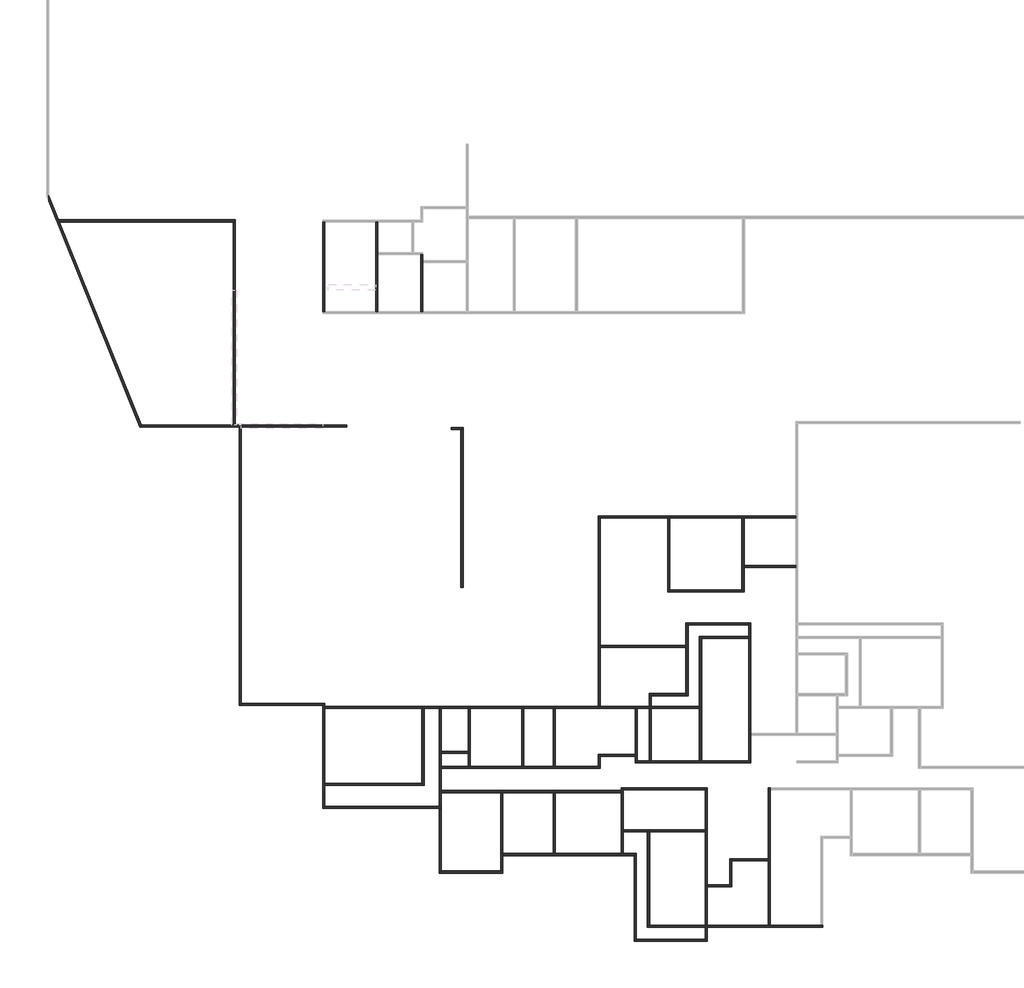
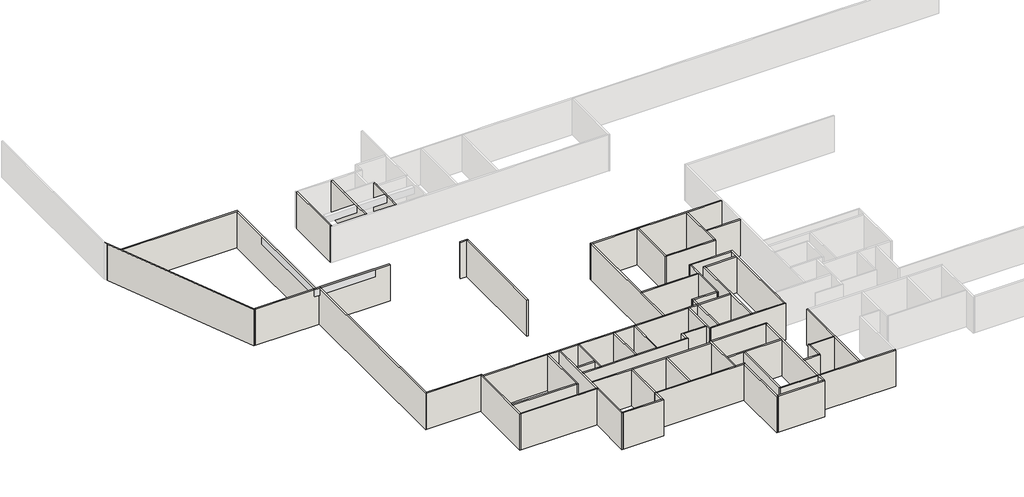
# One storey, part 1 of 8: 62 walls.
"""IFC4 building model written with IfcOpenShell, lengths in millimetres."""

from ifc_helpers import new_model, si_unit, origin, origin_with_axes, place, context, project, spatial, polyline, outline, extrude, faceted_brep, element, save

model = new_model("IFC4")

# Units and contexts
model_context = context("Model", 3, world=origin())
ifc_project = project(units=[si_unit("LENGTHUNIT", "METRE", prefix="MILLI")], contexts=[model_context])

# Site, building, storey
site = spatial("IfcSite", under=ifc_project)
building = spatial("IfcBuilding", under=site)
storey = spatial("IfcBuildingStorey", under=building, Name="户型图", Elevation=0.0)

# Walls
placement = place(None, origin())
element("IfcWall", 1, ObjectType="所有墙体", at=placement, inside=storey, context=model_context, shape_type="Brep", body=[
    faceted_brep([(85958.8477345, 57890.0043027, 0.0), (91177.79085, 44972.6668088, 0.0), (91177.79085, 44972.6668088, 3300.0), (85958.8477345, 57890.0043027, 3300.0), (85958.8477345, 58210.3403622, 0.0), (85958.8477345, 58210.3403622, 3300.0), (91258.731872, 45092.6668088, 3300.0), (91307.2150191, 44972.6668088, 3300.0), (91307.2150191, 44972.6668088, 0.0), (91258.731872, 45092.6668088, 0.0)], [[[0, 1, 2, 3]], [[4, 5, 6, 7, 8, 9]], [[1, 0, 4, 9, 8]], [[3, 2, 7, 6, 5]], [[0, 3, 5, 4]], [[2, 1, 8, 7]]]),
])
element("IfcWall", 2, ObjectType="所有墙体", at=placement, inside=storey, context=model_context, shape_type="Brep", body=[
    faceted_brep([(91307.2150191, 44972.6668088, 0.0), (96858.261361, 44972.6668088, 0.0), (96978.261361, 44972.6668088, 0.0), (96978.261361, 44972.6668088, 3300.0), (96858.261361, 44972.6668088, 3300.0), (96423.8477403, 44972.6668088, 3300.0), (91307.2150191, 44972.6668088, 3300.0), (91258.731872, 45092.6668088, 0.0), (91258.731872, 45092.6668088, 3300.0), (96723.8477403, 45092.6668088, 3300.0), (96978.261361, 45092.6668088, 3300.0), (96978.261361, 45092.6668088, 2700.0), (96978.261361, 45092.6668088, 0.0)], [[[0, 1, 2, 3, 4, 5, 6]], [[7, 8, 9, 10, 11, 12]], [[2, 1, 0, 7, 12]], [[6, 5, 4, 3, 10, 9, 8]], [[0, 6, 8, 7]], [[3, 2, 12, 11, 10]]]),
])
element("IfcWall", 3, ObjectType="所有墙体", at=placement, inside=storey, context=model_context, shape_type="Brep", body=[
    faceted_brep([(96858.261361, 44972.6668088, 0.0), (96858.261361, 29031.649632, 0.0), (96858.261361, 29031.649632, 3300.0), (96858.261361, 44882.6668088, 3300.0), (96858.261361, 44972.6668088, 3300.0), (96858.261361, 44972.6668088, 2700.0), (96978.261361, 44972.6668088, 0.0), (96978.261361, 44972.6668088, 3300.0), (96978.261361, 44882.6668088, 3300.0), (96978.261361, 29151.649632, 3300.0), (96978.261361, 29031.649632, 3300.0), (96978.261361, 29031.649632, 0.0), (96978.261361, 29151.649632, 0.0)], [[[0, 1, 2, 3, 4, 5]], [[6, 7, 8, 9, 10, 11, 12]], [[1, 0, 6, 12, 11]], [[4, 3, 2, 10, 9, 8, 7]], [[0, 5, 4, 7, 6]], [[2, 1, 11, 10]]]),
])
element("IfcWall", 4, ObjectType="所有墙体", at=placement, inside=storey, context=model_context, shape_type="Brep", body=[
    faceted_brep([(96978.261361, 29031.649632, 0.0), (101638.8477432, 29031.649632, 0.0), (101758.8477432, 29031.649632, 0.0), (101758.8477432, 29031.649632, 3300.0), (101638.8477432, 29031.649632, 3300.0), (96978.261361, 29031.649632, 3300.0), (96978.261361, 29151.649632, 0.0), (96978.261361, 29151.649632, 3300.0), (101648.7128309, 29151.649632, 3300.0), (101758.8477432, 29151.649632, 3300.0), (101758.8477432, 29151.649632, 2700.0), (101758.8477432, 29151.649632, 0.0)], [[[0, 1, 2, 3, 4, 5]], [[6, 7, 8, 9, 10, 11]], [[2, 1, 0, 6, 11]], [[5, 4, 3, 9, 8, 7]], [[0, 5, 7, 6]], [[3, 2, 11, 10, 9]]]),
])
element("IfcWall", 5, ObjectType="所有墙体", at=placement, inside=storey, context=model_context, shape_type="Brep", body=[
    faceted_brep([(101638.8477432, 29031.649632, 0.0), (101638.8477432, 23156.649475, 0.0), (101638.8477432, 23156.649475, 3300.0), (101638.8477432, 29031.649632, 3300.0), (101758.8477432, 29031.649632, 0.0), (101758.8477432, 29031.649632, 3300.0), (101758.8477432, 28766.8473862, 3300.0), (101758.8477432, 23276.649475, 3300.0), (101758.8477432, 23156.649475, 3300.0), (101758.8477432, 23156.649475, 0.0), (101758.8477432, 23276.649475, 0.0)], [[[0, 1, 2, 3]], [[4, 5, 6, 7, 8, 9, 10]], [[1, 0, 4, 10, 9]], [[3, 2, 8, 7, 6, 5]], [[0, 3, 5, 4]], [[2, 1, 9, 8]]]),
])
element("IfcWall", 6, ObjectType="所有墙体", at=placement, inside=storey, context=model_context, shape_type="Brep", body=[
    faceted_brep([(101758.8477432, 23156.649475, 0.0), (108307.9809936, 23156.649475, 0.0), (108427.9809936, 23156.649475, 0.0), (108427.9809936, 23156.649475, 3300.0), (108307.9809936, 23156.649475, 3300.0), (101758.8477432, 23156.649475, 3300.0), (101758.8477432, 23276.649475, 0.0), (101758.8477432, 23276.649475, 3300.0), (108427.9809936, 23276.649475, 3300.0), (108427.9809936, 23276.649475, 0.0)], [[[0, 1, 2, 3, 4, 5]], [[6, 7, 8, 9]], [[2, 1, 0, 6, 9]], [[5, 4, 3, 8, 7]], [[0, 5, 7, 6]], [[3, 2, 9, 8]]]),
])
element("IfcWall", 7, ObjectType="所有墙体", at=placement, inside=storey, context=model_context, shape_type="Brep", body=[
    faceted_brep([(108307.9809936, 23156.649475, 0.0), (108307.9809936, 19445.6854089, 0.0), (108307.9809936, 19445.6854089, 3300.0), (108307.9809936, 23156.649475, 3300.0), (108427.9809936, 23156.649475, 0.0), (108427.9809936, 23156.649475, 3300.0), (108427.9809936, 19565.6854089, 3300.0), (108427.9809936, 19445.6854089, 3300.0), (108427.9809936, 19445.6854089, 0.0), (108427.9809936, 19565.6854089, 0.0)], [[[0, 1, 2, 3]], [[4, 5, 6, 7, 8, 9]], [[1, 0, 4, 9, 8]], [[3, 2, 7, 6, 5]], [[0, 3, 5, 4]], [[2, 1, 8, 7]]]),
])
element("IfcWall", 8, ObjectType="所有墙体", at=placement, inside=storey, context=model_context, shape_type="Brep", body=[
    faceted_brep([(108427.9809936, 19445.6854089, 0.0), (111927.9809917, 19445.6854089, 0.0), (111927.9809917, 19445.6854089, 3300.0), (108427.9809936, 19445.6854089, 3300.0), (108427.9809936, 19565.6854089, 0.0), (108427.9809936, 19565.6854089, 3300.0), (111807.9809917, 19565.6854089, 3300.0), (111927.9809917, 19565.6854089, 3300.0), (111927.9809917, 19565.6854089, 0.0), (111807.9809917, 19565.6854089, 0.0)], [[[0, 1, 2, 3]], [[4, 5, 6, 7, 8, 9]], [[1, 0, 4, 9, 8]], [[3, 2, 7, 6, 5]], [[0, 3, 5, 4]], [[2, 1, 8, 7]]]),
])
element("IfcWall", 9, ObjectType="所有墙体", at=placement, inside=storey, context=model_context, shape_type="Brep", body=[
    faceted_brep([(111927.9809917, 19565.6854089, 0.0), (111927.9809917, 20445.6854086, 0.0), (111927.9809917, 20565.6854086, 0.0), (111927.9809917, 20565.6854086, 3300.0), (111927.9809917, 20445.6854086, 3300.0), (111927.9809917, 19565.6854089, 3300.0), (111807.9809917, 19565.6854089, 0.0), (111807.9809917, 19565.6854089, 3300.0), (111807.9809917, 20565.6854086, 3300.0), (111807.9809917, 20565.6854086, 0.0)], [[[0, 1, 2, 3, 4, 5]], [[6, 7, 8, 9]], [[2, 1, 0, 6, 9]], [[5, 4, 3, 8, 7]], [[0, 5, 7, 6]], [[3, 2, 9, 8]]]),
])
element("IfcWall", 10, ObjectType="所有墙体", at=placement, inside=storey, context=model_context, shape_type="Brep", body=[
    faceted_brep([(111927.9809917, 20445.6854086, 0.0), (119457.980985, 20445.6854086, 0.0), (119577.980985, 20445.6854086, 0.0), (119577.980985, 20445.6854086, 3300.0), (119457.980985, 20445.6854086, 3300.0), (111927.9809917, 20445.6854086, 3300.0), (111927.9809917, 20565.6854086, 0.0), (111927.9809917, 20565.6854086, 3300.0), (119577.980985, 20565.6854086, 3300.0), (119577.980985, 20565.6854086, 0.0)], [[[0, 1, 2, 3, 4, 5]], [[6, 7, 8, 9]], [[2, 1, 0, 6, 9]], [[5, 4, 3, 8, 7]], [[0, 5, 7, 6]], [[3, 2, 9, 8]]]),
])
element("IfcWall", 11, ObjectType="所有墙体", at=placement, inside=storey, context=model_context, shape_type="Brep", body=[
    faceted_brep([(119457.980985, 20445.6854086, 0.0), (119457.980985, 15545.6854122, 0.0), (119457.980985, 15545.6854122, 3300.0), (119457.980985, 20445.6854086, 3300.0), (119577.980985, 20445.6854086, 0.0), (119577.980985, 20445.6854086, 3300.0), (119577.980985, 15665.6854122, 3300.0), (119577.980985, 15545.6854122, 3300.0), (119577.980985, 15545.6854122, 0.0), (119577.980985, 15665.6854122, 0.0)], [[[0, 1, 2, 3]], [[4, 5, 6, 7, 8, 9]], [[1, 0, 4, 9, 8]], [[3, 2, 7, 6, 5]], [[0, 3, 5, 4]], [[2, 1, 8, 7]]]),
])
element("IfcWall", 12, ObjectType="所有墙体", at=placement, inside=storey, context=model_context, shape_type="Brep", body=[
    faceted_brep([(119577.980985, 15545.6854122, 0.0), (123627.9809864, 15545.6854122, 0.0), (123627.9809864, 15545.6854122, 3300.0), (119577.980985, 15545.6854122, 3300.0), (119577.980985, 15665.6854122, 0.0), (119577.980985, 15665.6854122, 3300.0), (123507.9809864, 15665.6854122, 3300.0), (123627.9809864, 15665.6854122, 3300.0), (123627.9809864, 15665.6854122, 0.0), (123507.9809864, 15665.6854122, 0.0)], [[[0, 1, 2, 3]], [[4, 5, 6, 7, 8, 9]], [[1, 0, 4, 9, 8]], [[3, 2, 7, 6, 5]], [[0, 3, 5, 4]], [[2, 1, 8, 7]]]),
])
element("IfcWall", 13, ObjectType="所有墙体", at=placement, inside=storey, context=model_context, shape_type="Brep", body=[
    faceted_brep([(123627.9809864, 15665.6854122, 0.0), (123627.9809864, 16345.6854162, 0.0), (123627.9809864, 16465.6854162, 0.0), (123627.9809864, 16465.6854162, 3300.0), (123627.9809864, 16345.6854162, 3300.0), (123627.9809864, 15665.6854122, 3300.0), (123507.9809864, 15665.6854122, 0.0), (123507.9809864, 15665.6854122, 3300.0), (123507.9809864, 16465.6854162, 3300.0), (123507.9809864, 16465.6854162, 0.0)], [[[0, 1, 2, 3, 4, 5]], [[6, 7, 8, 9]], [[2, 1, 0, 6, 9]], [[5, 4, 3, 8, 7]], [[0, 5, 7, 6]], [[3, 2, 9, 8]]]),
])
element("IfcWall", 14, ObjectType="所有墙体", at=placement, inside=storey, context=model_context, shape_type="Brep", body=[
    faceted_brep([(123627.9809864, 16345.6854162, 0.0), (130227.9809927, 16345.6854162, 0.0), (130227.9809927, 16345.6854162, 3300.0), (123627.9809864, 16345.6854162, 3300.0), (123627.9809864, 16465.6854162, 0.0), (123627.9809864, 16465.6854162, 3300.0), (130107.9809927, 16465.6854162, 3300.0), (130227.9809927, 16465.6854162, 3300.0), (130227.9809927, 16465.6854162, 0.0), (130107.9809927, 16465.6854162, 0.0)], [[[0, 1, 2, 3]], [[4, 5, 6, 7, 8, 9]], [[1, 0, 4, 9, 8]], [[3, 2, 7, 6, 5]], [[0, 3, 5, 4]], [[2, 1, 8, 7]]]),
])
element("IfcWall", 15, ObjectType="所有墙体", at=placement, inside=storey, context=model_context, shape_type="Brep", body=[
    faceted_brep([(128682.9654795, 39876.8473862, 0.0), (117388.847733, 39876.8473862, 0.0), (117388.847733, 39876.8473862, 3300.0), (128682.9654795, 39876.8473862, 3300.0), (128682.9654795, 39756.8473862, 0.0), (128682.9654795, 39756.8473862, 3300.0), (125733.822645, 39756.8473862, 3300.0), (125613.822645, 39756.8473862, 3300.0), (121483.5152585, 39756.8473862, 3300.0), (121363.5152585, 39756.8473862, 3300.0), (117508.847733, 39756.8473862, 3300.0), (117388.847733, 39756.8473862, 3300.0), (117388.847733, 39756.8473862, 0.0), (117508.847733, 39756.8473862, 0.0), (121363.5152585, 39756.8473862, 0.0), (121483.5152585, 39756.8473862, 0.0), (125613.822645, 39756.8473862, 0.0), (125733.822645, 39756.8473862, 0.0)], [[[0, 1, 2, 3]], [[4, 5, 6, 7, 8, 9, 10, 11, 12, 13, 14, 15, 16, 17]], [[1, 0, 4, 17, 16, 15, 14, 13, 12]], [[3, 2, 11, 10, 9, 8, 7, 6, 5]], [[0, 3, 5, 4]], [[2, 1, 12, 11]]]),
])
element("IfcWall", 16, ObjectType="所有墙体", at=placement, inside=storey, context=model_context, shape_type="Brep", body=[
    faceted_brep([(117388.847733, 39756.8473862, 0.0), (117388.847733, 28976.8473862, 0.0), (117388.847733, 28976.8473862, 3300.0), (117388.847733, 39756.8473862, 3300.0), (117508.847733, 39756.8473862, 0.0), (117508.847733, 39756.8473862, 3300.0), (117508.847733, 32476.6854027, 3300.0), (117508.847733, 32356.6854027, 3300.0), (117508.847733, 28976.8473862, 3300.0), (117508.847733, 28976.8473862, 0.0), (117508.847733, 32356.6854027, 0.0), (117508.847733, 32476.6854027, 0.0)], [[[0, 1, 2, 3]], [[4, 5, 6, 7, 8, 9, 10, 11]], [[1, 0, 4, 11, 10, 9]], [[3, 2, 8, 7, 6, 5]], [[0, 3, 5, 4]], [[2, 1, 9, 8]]]),
])
element("IfcWall", 17, ObjectType="所有墙体", at=placement, inside=storey, context=model_context, shape_type="Brep", body=[
    faceted_brep([(123182.9809894, 28976.8473862, 0.0), (120427.9809941, 28976.8473862, 0.0), (120307.9809941, 28976.8473862, 0.0), (117508.847733, 28976.8473862, 0.0), (117388.847733, 28976.8473862, 0.0), (101758.8477432, 28976.8473862, 0.0), (101758.8477432, 28976.8473862, 3300.0), (117388.847733, 28976.8473862, 3300.0), (117508.847733, 28976.8473862, 3300.0), (120307.9809941, 28976.8473862, 3300.0), (120427.9809941, 28976.8473862, 3300.0), (123182.9809894, 28976.8473862, 3300.0), (123182.9809894, 28856.8473862, 0.0), (123182.9809894, 28856.8473862, 3300.0), (120427.9809941, 28856.8473862, 3300.0), (120307.9809941, 28856.8473862, 3300.0), (119627.9809584, 28856.8473862, 3300.0), (119507.9809584, 28856.8473862, 3300.0), (114927.98099, 28856.8473862, 3300.0), (114807.98099, 28856.8473862, 3300.0), (113127.9809937, 28856.8473862, 3300.0), (113007.9809937, 28856.8473862, 3300.0), (110077.7500653, 28856.8473862, 3300.0), (109957.7500653, 28856.8473862, 3300.0), (108427.9809936, 28856.8473862, 3300.0), (108307.9809936, 28856.8473862, 3300.0), (107427.9809842, 28856.8473862, 3300.0), (107307.9809842, 28856.8473862, 3300.0), (101758.8477432, 28856.8473862, 3300.0), (101758.8477432, 28856.8473862, 0.0), (107307.9809842, 28856.8473862, 0.0), (107427.9809842, 28856.8473862, 0.0), (108307.9809936, 28856.8473862, 0.0), (108427.9809936, 28856.8473862, 0.0), (109957.7500653, 28856.8473862, 0.0), (110077.7500653, 28856.8473862, 0.0), (113007.9809937, 28856.8473862, 0.0), (113127.9809937, 28856.8473862, 0.0), (114807.98099, 28856.8473862, 0.0), (114927.98099, 28856.8473862, 0.0), (119507.9809584, 28856.8473862, 0.0), (119627.9809584, 28856.8473862, 0.0), (120307.9809941, 28856.8473862, 0.0), (120427.9809941, 28856.8473862, 0.0)], [[[0, 1, 2, 3, 4, 5, 6, 7, 8, 9, 10, 11]], [[12, 13, 14, 15, 16, 17, 18, 19, 20, 21, 22, 23, 24, 25, 26, 27, 28, 29, 30, 31, 32, 33, 34, 35, 36, 37, 38, 39, 40, 41, 42, 43]], [[5, 4, 3, 2, 1, 0, 12, 43, 42, 41, 40, 39, 38, 37, 36, 35, 34, 33, 32, 31, 30, 29]], [[11, 10, 9, 8, 7, 6, 28, 27, 26, 25, 24, 23, 22, 21, 20, 19, 18, 17, 16, 15, 14, 13]], [[6, 5, 29, 28]], [[0, 11, 13, 12]]]),
])
element("IfcWall", 18, ObjectType="所有墙体", at=placement, inside=storey, context=model_context, shape_type="Brep", body=[
    faceted_brep([(86566.2983649, 56706.847293, 0.0), (96513.8477403, 56706.847293, 0.0), (96633.8477403, 56706.847293, 0.0), (96633.8477403, 56706.847293, 3300.0), (96513.8477403, 56706.847293, 3300.0), (86566.2983649, 56706.847293, 3300.0), (86517.8152178, 56826.847293, 0.0), (86517.8152178, 56826.847293, 3300.0), (96633.8477403, 56826.847293, 3300.0), (96633.8477403, 56826.847293, 0.0)], [[[0, 1, 2, 3, 4, 5]], [[6, 7, 8, 9]], [[2, 1, 0, 6, 9]], [[5, 4, 3, 8, 7]], [[0, 5, 7, 6]], [[3, 2, 9, 8]]]),
])
element("IfcWall", 19, ObjectType="所有墙体", at=placement, inside=storey, context=model_context, shape_type="SweptSolid", body=[
    extrude(outline(polyline([(96513.8477403, 45092.6668088), (96513.8477403, 56706.847293), (96633.8477403, 56706.847293), (96633.8477403, 45092.6668088), (96513.8477403, 45092.6668088)])), origin_with_axes(), (0.0, 0.0, 1.0), 3300.0),
])
element("IfcWall", 20, ObjectType="所有墙体", at=placement, inside=storey, context=model_context, shape_type="Brep", body=[
    faceted_brep([(101758.8477337, 51576.8472247, 0.0), (101758.8477337, 56681.8460485, 0.0), (101758.8477337, 56681.8460485, 2700.0), (101758.8477337, 56681.8460485, 3300.0), (101758.8477337, 53116.9449825, 3300.0), (101758.8477337, 52816.9449825, 3300.0), (101758.8477337, 51576.8472247, 3300.0), (101758.8477337, 51576.8472247, 2700.0), (101638.8477337, 51576.8472247, 0.0), (101638.8477337, 51576.8472247, 3300.0), (101638.8477337, 52816.9449825, 3300.0), (101638.8477337, 53116.9449825, 3300.0), (101638.8477337, 56681.8460485, 3300.0), (101638.8477337, 56681.8460485, 0.0)], [[[0, 1, 2, 3, 4, 5, 6, 7]], [[8, 9, 10, 11, 12, 13]], [[1, 0, 8, 13]], [[6, 5, 4, 3, 12, 11, 10, 9]], [[3, 2, 1, 13, 12]], [[0, 7, 6, 9, 8]]]),
])
element("IfcWall", 21, ObjectType="所有墙体", at=placement, inside=storey, context=model_context, shape_type="Brep", body=[
    faceted_brep([(104655.6151291, 56681.8460485, 0.0), (104655.6151291, 51576.8472247, 0.0), (104655.6151291, 51576.8472247, 3300.0), (104655.6151291, 52816.9449825, 3300.0), (104655.6151291, 53116.9449825, 3300.0), (104655.6151291, 56681.8460485, 3300.0), (104775.6151291, 56681.8460485, 0.0), (104775.6151291, 56681.8460485, 3300.0), (104775.6151291, 54951.5480835, 3300.0), (104775.6151291, 54831.5480835, 3300.0), (104775.6151291, 53116.9449825, 3300.0), (104775.6151291, 52816.9449825, 3300.0), (104775.6151291, 51576.8472247, 3300.0), (104775.6151291, 51576.8472247, 0.0), (104775.6151291, 54831.5480835, 0.0), (104775.6151291, 54951.5480835, 0.0)], [[[0, 1, 2, 3, 4, 5]], [[6, 7, 8, 9, 10, 11, 12, 13, 14, 15]], [[1, 0, 6, 15, 14, 13]], [[5, 4, 3, 2, 12, 11, 10, 9, 8, 7]], [[0, 5, 7, 6]], [[2, 1, 13, 12]]]),
])
element("IfcWall", 22, ObjectType="所有墙体", at=placement, inside=storey, context=model_context, shape_type="Brep", body=[
    faceted_brep([(107238.8477337, 54831.5480835, 0.0), (107238.8477337, 51576.8472247, 0.0), (107238.8477337, 51576.8472247, 3300.0), (107238.8477337, 52816.9449825, 3300.0), (107238.8477337, 53116.9449825, 3300.0), (107238.8477337, 54831.5480835, 3300.0), (107358.8477337, 54831.5480835, 0.0), (107358.8477337, 54831.5480835, 3300.0), (107358.8477337, 54487.0649839, 3300.0), (107358.8477337, 54367.0649839, 3300.0), (107358.8477337, 53116.9449825, 3300.0), (107358.8477337, 52816.9449825, 3300.0), (107358.8477337, 51576.8472247, 3300.0), (107358.8477337, 51576.8472247, 0.0), (107358.8477337, 54367.0649839, 0.0), (107358.8477337, 54487.0649839, 0.0)], [[[0, 1, 2, 3, 4, 5]], [[6, 7, 8, 9, 10, 11, 12, 13, 14, 15]], [[1, 0, 6, 15, 14, 13]], [[5, 4, 3, 2, 12, 11, 10, 9, 8, 7]], [[0, 5, 7, 6]], [[2, 1, 13, 12]]]),
])
element("IfcWall", 23, ObjectType="所有墙体", at=placement, inside=storey, context=model_context, shape_type="SweptSolid", body=[
    extrude(outline(polyline([(96978.261361, 45092.6668088), (102998.8477404, 45092.6668088), (102998.8477404, 44972.6668088), (96978.261361, 44972.6668088), (96978.261361, 45092.6668088)])), origin_with_axes(), (0.0, 0.0, 1.0), 3300.0),
])
element("IfcWall", 24, ObjectType="所有墙体", at=placement, inside=storey, context=model_context, shape_type="Brep", body=[
    faceted_brep([(108998.8477274, 44831.6496338, 0.0), (109538.8477346, 44831.6496338, 0.0), (109658.8477346, 44831.6496338, 0.0), (109658.8477346, 44831.6496338, 3300.0), (109538.8477346, 44831.6496338, 3300.0), (108998.8477274, 44831.6496338, 3300.0), (108998.8477274, 44951.6496338, 0.0), (108998.8477274, 44951.6496338, 3300.0), (109658.8477346, 44951.6496338, 3300.0), (109658.8477346, 44951.6496338, 0.0)], [[[0, 1, 2, 3, 4, 5]], [[6, 7, 8, 9]], [[2, 1, 0, 6, 9]], [[5, 4, 3, 8, 7]], [[0, 5, 7, 6]], [[3, 2, 9, 8]]]),
])
element("IfcWall", 25, ObjectType="所有墙体", at=placement, inside=storey, context=model_context, shape_type="SweptSolid", body=[
    extrude(outline(polyline([(109538.8477346, 35791.6496371), (109538.8477346, 44831.6496338), (109658.8477346, 44831.6496338), (109658.8477346, 35791.6496371), (109538.8477346, 35791.6496371)])), origin_with_axes(), (0.0, 0.0, 1.0), 3300.0),
])
element("IfcWall", 26, ObjectType="所有墙体", at=placement, inside=storey, context=model_context, shape_type="Brep", body=[
    faceted_brep([(107307.9809842, 28856.8473862, 0.0), (107307.9809842, 24576.6494805, 0.0), (107307.9809842, 24456.6494805, 0.0), (107307.9809842, 24456.6494805, 3300.0), (107307.9809842, 24576.6494805, 3300.0), (107307.9809842, 28856.8473862, 3300.0), (107427.9809842, 28856.8473862, 0.0), (107427.9809842, 28856.8473862, 3300.0), (107427.9809842, 24456.6494805, 3300.0), (107427.9809842, 24456.6494805, 0.0)], [[[0, 1, 2, 3, 4, 5]], [[6, 7, 8, 9]], [[2, 1, 0, 6, 9]], [[5, 4, 3, 8, 7]], [[0, 5, 7, 6]], [[3, 2, 9, 8]]]),
])
element("IfcWall", 27, ObjectType="所有墙体", at=placement, inside=storey, context=model_context, shape_type="SweptSolid", body=[
    extrude(outline(polyline([(101758.8477432, 24576.6494805), (107307.9809842, 24576.6494805), (107307.9809842, 24456.6494805), (101758.8477432, 24456.6494805), (101758.8477432, 24576.6494805)])), origin_with_axes(), (0.0, 0.0, 1.0), 3300.0),
])
element("IfcWall", 28, ObjectType="所有墙体", at=placement, inside=storey, context=model_context, shape_type="Brep", body=[
    faceted_brep([(108307.9809936, 28856.8473862, 0.0), (108307.9809936, 23276.649475, 0.0), (108307.9809936, 23276.649475, 3300.0), (108307.9809936, 28856.8473862, 3300.0), (108427.9809936, 28856.8473862, 0.0), (108427.9809936, 28856.8473862, 3300.0), (108427.9809936, 26415.6836281, 3300.0), (108427.9809936, 26295.6836281, 3300.0), (108427.9809936, 25565.6854178, 3300.0), (108427.9809936, 25445.6854178, 3300.0), (108427.9809936, 24166.1844489, 3300.0), (108427.9809936, 24046.1844489, 3300.0), (108427.9809936, 23276.649475, 3300.0), (108427.9809936, 23276.649475, 0.0), (108427.9809936, 24046.1844489, 0.0), (108427.9809936, 24166.1844489, 0.0), (108427.9809936, 25445.6854178, 0.0), (108427.9809936, 25565.6854178, 0.0), (108427.9809936, 26295.6836281, 0.0), (108427.9809936, 26415.6836281, 0.0)], [[[0, 1, 2, 3]], [[4, 5, 6, 7, 8, 9, 10, 11, 12, 13, 14, 15, 16, 17, 18, 19]], [[1, 0, 4, 19, 18, 17, 16, 15, 14, 13]], [[3, 2, 12, 11, 10, 9, 8, 7, 6, 5]], [[2, 1, 13, 12]], [[0, 3, 5, 4]]]),
])
element("IfcWall", 29, ObjectType="所有墙体", at=placement, inside=storey, context=model_context, shape_type="SweptSolid", body=[
    extrude(outline(polyline([(109957.7500653, 26295.6836281), (108427.9809936, 26295.6836281), (108427.9809936, 26415.6836281), (109957.7500653, 26415.6836281), (109957.7500653, 26295.6836281)])), origin_with_axes(), (0.0, 0.0, 1.0), 3300.0),
])
element("IfcWall", 30, ObjectType="所有墙体", at=placement, inside=storey, context=model_context, shape_type="Brep", body=[
    faceted_brep([(110077.7500653, 25565.6854178, 0.0), (110077.7500653, 28856.8473862, 0.0), (110077.7500653, 28856.8473862, 3300.0), (110077.7500653, 25565.6854178, 3300.0), (109957.7500653, 25565.6854178, 0.0), (109957.7500653, 25565.6854178, 3300.0), (109957.7500653, 26295.6836281, 3300.0), (109957.7500653, 26415.6836281, 3300.0), (109957.7500653, 28856.8473862, 3300.0), (109957.7500653, 28856.8473862, 0.0), (109957.7500653, 26415.6836281, 0.0), (109957.7500653, 26295.6836281, 0.0)], [[[0, 1, 2, 3]], [[4, 5, 6, 7, 8, 9, 10, 11]], [[1, 0, 4, 11, 10, 9]], [[3, 2, 8, 7, 6, 5]], [[2, 1, 9, 8]], [[0, 3, 5, 4]]]),
])
element("IfcWall", 31, ObjectType="所有墙体", at=placement, inside=storey, context=model_context, shape_type="Brep", body=[
    faceted_brep([(117508.847733, 25565.6854178, 0.0), (117388.847733, 25565.6854178, 0.0), (114927.98099, 25565.6854178, 0.0), (114807.98099, 25565.6854178, 0.0), (113127.9809937, 25565.6854178, 0.0), (113007.9809937, 25565.6854178, 0.0), (110077.7500653, 25565.6854178, 0.0), (109957.7500653, 25565.6854178, 0.0), (108427.9809936, 25565.6854178, 0.0), (108427.9809936, 25565.6854178, 3300.0), (109957.7500653, 25565.6854178, 3300.0), (110077.7500653, 25565.6854178, 3300.0), (113007.9809937, 25565.6854178, 3300.0), (113127.9809937, 25565.6854178, 3300.0), (114807.98099, 25565.6854178, 3300.0), (114927.98099, 25565.6854178, 3300.0), (117388.847733, 25565.6854178, 3300.0), (117508.847733, 25565.6854178, 3300.0), (117508.847733, 25445.6854178, 0.0), (117508.847733, 25445.6854178, 3300.0), (108427.9809936, 25445.6854178, 3300.0), (108427.9809936, 25445.6854178, 0.0)], [[[0, 1, 2, 3, 4, 5, 6, 7, 8, 9, 10, 11, 12, 13, 14, 15, 16, 17]], [[18, 19, 20, 21]], [[8, 7, 6, 5, 4, 3, 2, 1, 0, 18, 21]], [[17, 16, 15, 14, 13, 12, 11, 10, 9, 20, 19]], [[9, 8, 21, 20]], [[0, 17, 19, 18]]]),
])
element("IfcWall", 32, ObjectType="所有墙体", at=placement, inside=storey, context=model_context, shape_type="Brep", body=[
    faceted_brep([(117508.847733, 25565.6854178, 0.0), (117508.847733, 26125.3729134, 0.0), (117508.847733, 26245.3729134, 0.0), (117508.847733, 26245.3729134, 3300.0), (117508.847733, 26125.3729134, 3300.0), (117508.847733, 25565.6854178, 3300.0), (117388.847733, 25565.6854178, 0.0), (117388.847733, 25565.6854178, 3300.0), (117388.847733, 26245.3729134, 3300.0), (117388.847733, 26245.3729134, 0.0)], [[[0, 1, 2, 3, 4, 5]], [[6, 7, 8, 9]], [[2, 1, 0, 6, 9]], [[5, 4, 3, 8, 7]], [[0, 5, 7, 6]], [[3, 2, 9, 8]]]),
])
element("IfcWall", 33, ObjectType="所有墙体", at=placement, inside=storey, context=model_context, shape_type="SweptSolid", body=[
    extrude(outline(polyline([(119507.9809584, 26125.3729134), (117508.847733, 26125.3729134), (117508.847733, 26245.3729134), (119507.9809584, 26245.3729134), (119507.9809584, 26125.3729134)])), origin_with_axes(), (0.0, 0.0, 1.0), 3300.0),
])
element("IfcWall", 34, ObjectType="所有墙体", at=placement, inside=storey, context=model_context, shape_type="Brep", body=[
    faceted_brep([(119627.9809584, 25746.1844435, 0.0), (119627.9809584, 25866.1844435, 0.0), (119627.9809584, 28856.8473862, 0.0), (119627.9809584, 28856.8473862, 3300.0), (119627.9809584, 25866.1844435, 3300.0), (119627.9809584, 25746.1844435, 3300.0), (119507.9809584, 25746.1844435, 0.0), (119507.9809584, 25746.1844435, 3300.0), (119507.9809584, 26125.3729134, 3300.0), (119507.9809584, 26245.3729134, 3300.0), (119507.9809584, 28856.8473862, 3300.0), (119507.9809584, 28856.8473862, 0.0), (119507.9809584, 26245.3729134, 0.0), (119507.9809584, 26125.3729134, 0.0)], [[[0, 1, 2, 3, 4, 5]], [[6, 7, 8, 9, 10, 11, 12, 13]], [[2, 1, 0, 6, 13, 12, 11]], [[5, 4, 3, 10, 9, 8, 7]], [[3, 2, 11, 10]], [[0, 5, 7, 6]]]),
])
element("IfcWall", 35, ObjectType="所有墙体", at=placement, inside=storey, context=model_context, shape_type="SweptSolid", body=[
    extrude(outline(polyline([(113007.9809937, 25565.6854178), (113007.9809937, 28856.8473862), (113127.9809937, 28856.8473862), (113127.9809937, 25565.6854178), (113007.9809937, 25565.6854178)])), origin_with_axes(), (0.0, 0.0, 1.0), 3300.0),
])
element("IfcWall", 36, ObjectType="所有墙体", at=placement, inside=storey, context=model_context, shape_type="SweptSolid", body=[
    extrude(outline(polyline([(114807.98099, 25565.6854178), (114807.98099, 28856.8473862), (114927.98099, 28856.8473862), (114927.98099, 25565.6854178), (114807.98099, 25565.6854178)])), origin_with_axes(), (0.0, 0.0, 1.0), 3300.0),
])
element("IfcWall", 37, ObjectType="所有墙体", at=placement, inside=storey, context=model_context, shape_type="Brep", body=[
    faceted_brep([(119627.9809584, 25746.1844435, 0.0), (126127.9809859, 25746.1844435, 0.0), (126127.9809859, 25746.1844435, 3300.0), (119627.9809584, 25746.1844435, 3300.0), (119627.9809584, 25866.1844435, 0.0), (119627.9809584, 25866.1844435, 3300.0), (120307.9809941, 25866.1844435, 3300.0), (120427.9809941, 25866.1844435, 3300.0), (123182.9809894, 25866.1844435, 3300.0), (123302.9809894, 25866.1844435, 3300.0), (126007.9809859, 25866.1844435, 3300.0), (126127.9809859, 25866.1844435, 3300.0), (126127.9809859, 25866.1844435, 0.0), (126007.9809859, 25866.1844435, 0.0), (123302.9809894, 25866.1844435, 0.0), (123182.9809894, 25866.1844435, 0.0), (120427.9809941, 25866.1844435, 0.0), (120307.9809941, 25866.1844435, 0.0)], [[[0, 1, 2, 3]], [[4, 5, 6, 7, 8, 9, 10, 11, 12, 13, 14, 15, 16, 17]], [[1, 0, 4, 17, 16, 15, 14, 13, 12]], [[3, 2, 11, 10, 9, 8, 7, 6, 5]], [[0, 3, 5, 4]], [[2, 1, 12, 11]]]),
])
element("IfcWall", 38, ObjectType="所有墙体", at=placement, inside=storey, context=model_context, shape_type="Brep", body=[
    faceted_brep([(126127.9809859, 25866.1844435, 0.0), (126127.9809859, 27331.6496402, 0.0), (126127.9809859, 27451.6496402, 0.0), (126127.9809859, 33765.6854157, 0.0), (126127.9809859, 33765.6854157, 3300.0), (126127.9809859, 27451.6496402, 3300.0), (126127.9809859, 27331.6496402, 3300.0), (126127.9809859, 25866.1844435, 3300.0), (126007.9809859, 25866.1844435, 0.0), (126007.9809859, 25866.1844435, 3300.0), (126007.9809859, 32870.685413, 3300.0), (126007.9809859, 32990.685413, 3300.0), (126007.9809859, 33645.6854157, 3300.0), (126007.9809859, 33765.6854157, 3300.0), (126007.9809859, 33765.6854157, 0.0), (126007.9809859, 33645.6854157, 0.0), (126007.9809859, 32990.685413, 0.0), (126007.9809859, 32870.685413, 0.0)], [[[0, 1, 2, 3, 4, 5, 6, 7]], [[8, 9, 10, 11, 12, 13, 14, 15, 16, 17]], [[3, 2, 1, 0, 8, 17, 16, 15, 14]], [[7, 6, 5, 4, 13, 12, 11, 10, 9]], [[0, 7, 9, 8]], [[4, 3, 14, 13]]]),
])
element("IfcWall", 39, ObjectType="所有墙体", at=placement, inside=storey, context=model_context, shape_type="Brep", body=[
    faceted_brep([(126007.9809859, 33765.6854157, 0.0), (122407.9809949, 33765.6854157, 0.0), (122407.9809949, 33765.6854157, 3300.0), (126007.9809859, 33765.6854157, 3300.0), (126007.9809859, 33645.6854157, 0.0), (126007.9809859, 33645.6854157, 3300.0), (122527.9809949, 33645.6854157, 3300.0), (122407.9809949, 33645.6854157, 3300.0), (122407.9809949, 33645.6854157, 0.0), (122527.9809949, 33645.6854157, 0.0)], [[[0, 1, 2, 3]], [[4, 5, 6, 7, 8, 9]], [[1, 0, 4, 9, 8]], [[3, 2, 7, 6, 5]], [[0, 3, 5, 4]], [[2, 1, 8, 7]]]),
])
element("IfcWall", 40, ObjectType="所有墙体", at=placement, inside=storey, context=model_context, shape_type="Brep", body=[
    faceted_brep([(122407.9809949, 33645.6854157, 0.0), (122407.9809949, 32476.6854027, 0.0), (122407.9809949, 32356.6854027, 0.0), (122407.9809949, 29715.6854131, 0.0), (122407.9809949, 29595.6854131, 0.0), (122407.9809949, 29595.6854131, 3300.0), (122407.9809949, 29715.6854131, 3300.0), (122407.9809949, 32356.6854027, 3300.0), (122407.9809949, 32476.6854027, 3300.0), (122407.9809949, 33645.6854157, 3300.0), (122527.9809949, 33645.6854157, 0.0), (122527.9809949, 33645.6854157, 3300.0), (122527.9809949, 29595.6854131, 3300.0), (122527.9809949, 29595.6854131, 0.0)], [[[0, 1, 2, 3, 4, 5, 6, 7, 8, 9]], [[10, 11, 12, 13]], [[4, 3, 2, 1, 0, 10, 13]], [[9, 8, 7, 6, 5, 12, 11]], [[0, 9, 11, 10]], [[5, 4, 13, 12]]]),
])
element("IfcWall", 41, ObjectType="所有墙体", at=placement, inside=storey, context=model_context, shape_type="Brep", body=[
    faceted_brep([(122407.9809949, 29715.6854131, 0.0), (120307.9809941, 29715.6854131, 0.0), (120307.9809941, 29715.6854131, 3300.0), (122407.9809949, 29715.6854131, 3300.0), (122407.9809949, 29595.6854131, 0.0), (122407.9809949, 29595.6854131, 3300.0), (120427.9809941, 29595.6854131, 3300.0), (120307.9809941, 29595.6854131, 3300.0), (120307.9809941, 29595.6854131, 0.0), (120427.9809941, 29595.6854131, 0.0)], [[[0, 1, 2, 3]], [[4, 5, 6, 7, 8, 9]], [[1, 0, 4, 9, 8]], [[3, 2, 7, 6, 5]], [[0, 3, 5, 4]], [[2, 1, 8, 7]]]),
])
element("IfcWall", 42, ObjectType="所有墙体", at=placement, inside=storey, context=model_context, shape_type="SweptSolid", body=[
    extrude(outline(polyline([(120427.9809941, 25866.1844435), (120307.9809941, 25866.1844435), (120307.9809941, 28856.8473862), (120427.9809941, 28856.8473862), (120427.9809941, 25866.1844435)])), origin_with_axes(), (0.0, 0.0, 1.0), 3300.0),
    extrude(outline(polyline([(120307.9809941, 29595.6854131), (120427.9809941, 29595.6854131), (120427.9809941, 28976.8473862), (120307.9809941, 28976.8473862), (120307.9809941, 29595.6854131)])), origin_with_axes(), (0.0, 0.0, 1.0), 3300.0),
])
element("IfcWall", 43, ObjectType="所有墙体", at=placement, inside=storey, context=model_context, shape_type="Brep", body=[
    faceted_brep([(123302.9809894, 25866.1844435, 0.0), (123302.9809894, 32870.685413, 0.0), (123302.9809894, 32990.685413, 0.0), (123302.9809894, 32990.685413, 3300.0), (123302.9809894, 32870.685413, 3300.0), (123302.9809894, 25866.1844435, 3300.0), (123182.9809894, 25866.1844435, 0.0), (123182.9809894, 25866.1844435, 3300.0), (123182.9809894, 28856.8473862, 3300.0), (123182.9809894, 28976.8473862, 3300.0), (123182.9809894, 32990.685413, 3300.0), (123182.9809894, 32990.685413, 0.0), (123182.9809894, 28976.8473862, 0.0), (123182.9809894, 28856.8473862, 0.0)], [[[0, 1, 2, 3, 4, 5]], [[6, 7, 8, 9, 10, 11, 12, 13]], [[2, 1, 0, 6, 13, 12, 11]], [[5, 4, 3, 10, 9, 8, 7]], [[3, 2, 11, 10]], [[0, 5, 7, 6]]]),
])
element("IfcWall", 44, ObjectType="所有墙体", at=placement, inside=storey, context=model_context, shape_type="SweptSolid", body=[
    extrude(outline(polyline([(126007.9809859, 32870.685413), (123302.9809894, 32870.685413), (123302.9809894, 32990.685413), (126007.9809859, 32990.685413), (126007.9809859, 32870.685413)])), origin_with_axes(), (0.0, 0.0, 1.0), 3300.0),
])
element("IfcWall", 45, ObjectType="所有墙体", at=placement, inside=storey, context=model_context, shape_type="SweptSolid", body=[
    extrude(outline(polyline([(122407.9809949, 32356.6854027), (117508.847733, 32356.6854027), (117508.847733, 32476.6854027), (122407.9809949, 32476.6854027), (122407.9809949, 32356.6854027)])), origin_with_axes(), (0.0, 0.0, 1.0), 3300.0),
])
element("IfcWall", 46, ObjectType="所有墙体", at=placement, inside=storey, context=model_context, shape_type="Brep", body=[
    faceted_brep([(121363.5152585, 39756.8473862, 0.0), (121363.5152585, 35520.9842054, 0.0), (121363.5152585, 35520.9842054, 3300.0), (121363.5152585, 39756.8473862, 3300.0), (121483.5152585, 39756.8473862, 0.0), (121483.5152585, 39756.8473862, 3300.0), (121483.5152585, 35640.9842054, 3300.0), (121483.5152585, 35520.9842054, 3300.0), (121483.5152585, 35520.9842054, 0.0), (121483.5152585, 35640.9842054, 0.0)], [[[0, 1, 2, 3]], [[4, 5, 6, 7, 8, 9]], [[1, 0, 4, 9, 8]], [[3, 2, 7, 6, 5]], [[0, 3, 5, 4]], [[2, 1, 8, 7]]]),
])
element("IfcWall", 47, ObjectType="所有墙体", at=placement, inside=storey, context=model_context, shape_type="Brep", body=[
    faceted_brep([(121483.5152585, 35520.9842054, 0.0), (125733.822645, 35520.9842054, 0.0), (125733.822645, 35520.9842054, 3300.0), (121483.5152585, 35520.9842054, 3300.0), (121483.5152585, 35640.9842054, 0.0), (121483.5152585, 35640.9842054, 3300.0), (125613.822645, 35640.9842054, 3300.0), (125733.822645, 35640.9842054, 3300.0), (125733.822645, 35640.9842054, 0.0), (125613.822645, 35640.9842054, 0.0)], [[[0, 1, 2, 3]], [[4, 5, 6, 7, 8, 9]], [[1, 0, 4, 9, 8]], [[3, 2, 7, 6, 5]], [[0, 3, 5, 4]], [[2, 1, 8, 7]]]),
])
element("IfcWall", 48, ObjectType="所有墙体", at=placement, inside=storey, context=model_context, shape_type="Brep", body=[
    faceted_brep([(125733.822645, 35640.9842054, 0.0), (125733.822645, 36931.6496402, 0.0), (125733.822645, 37051.6496402, 0.0), (125733.822645, 39756.8473862, 0.0), (125733.822645, 39756.8473862, 3300.0), (125733.822645, 37051.6496402, 3300.0), (125733.822645, 36931.6496402, 3300.0), (125733.822645, 35640.9842054, 3300.0), (125613.822645, 35640.9842054, 0.0), (125613.822645, 35640.9842054, 3300.0), (125613.822645, 39756.8473862, 3300.0), (125613.822645, 39756.8473862, 0.0)], [[[0, 1, 2, 3, 4, 5, 6, 7]], [[8, 9, 10, 11]], [[3, 2, 1, 0, 8, 11]], [[7, 6, 5, 4, 10, 9]], [[0, 7, 9, 8]], [[4, 3, 11, 10]]]),
])
element("IfcWall", 49, ObjectType="所有墙体", at=placement, inside=storey, context=model_context, shape_type="SweptSolid", body=[
    extrude(outline(polyline([(128682.9654795, 36931.6496402), (125733.822645, 36931.6496402), (125733.822645, 37051.6496402), (128682.9654795, 37051.6496402), (128682.9654795, 36931.6496402)])), origin_with_axes(), (0.0, 0.0, 1.0), 3300.0),
])
element("IfcWall", 50, ObjectType="所有墙体", at=placement, inside=storey, context=model_context, shape_type="Brep", body=[
    faceted_brep([(108427.9809936, 24046.1844489, 0.0), (111807.9809917, 24046.1844489, 0.0), (111927.9809917, 24046.1844489, 0.0), (114807.98099, 24046.1844489, 0.0), (114927.98099, 24046.1844489, 0.0), (118707.9809885, 24046.1844489, 0.0), (118707.9809885, 24046.1844489, 3300.0), (114927.98099, 24046.1844489, 3300.0), (114807.98099, 24046.1844489, 3300.0), (111927.9809917, 24046.1844489, 3300.0), (111807.9809917, 24046.1844489, 3300.0), (108427.9809936, 24046.1844489, 3300.0), (108427.9809936, 24166.1844489, 0.0), (108427.9809936, 24166.1844489, 3300.0), (118707.9809885, 24166.1844489, 3300.0), (118707.9809885, 24166.1844489, 0.0)], [[[0, 1, 2, 3, 4, 5, 6, 7, 8, 9, 10, 11]], [[12, 13, 14, 15]], [[5, 4, 3, 2, 1, 0, 12, 15]], [[11, 10, 9, 8, 7, 6, 14, 13]], [[0, 11, 13, 12]], [[6, 5, 15, 14]]]),
])
element("IfcWall", 51, ObjectType="所有墙体", at=placement, inside=storey, context=model_context, shape_type="Brep", body=[
    faceted_brep([(118827.9809885, 20565.6854086, 0.0), (118827.9809885, 21796.1844471, 0.0), (118827.9809885, 21916.1844471, 0.0), (118827.9809885, 24196.1844453, 0.0), (118827.9809885, 24316.1844453, 0.0), (118827.9809885, 24316.1844453, 3300.0), (118827.9809885, 24196.1844453, 3300.0), (118827.9809885, 21916.1844471, 3300.0), (118827.9809885, 21796.1844471, 3300.0), (118827.9809885, 20565.6854086, 3300.0), (118707.9809885, 20565.6854086, 0.0), (118707.9809885, 20565.6854086, 3300.0), (118707.9809885, 24046.1844489, 3300.0), (118707.9809885, 24166.1844489, 3300.0), (118707.9809885, 24316.1844453, 3300.0), (118707.9809885, 24316.1844453, 0.0), (118707.9809885, 24166.1844489, 0.0), (118707.9809885, 24046.1844489, 0.0)], [[[0, 1, 2, 3, 4, 5, 6, 7, 8, 9]], [[10, 11, 12, 13, 14, 15, 16, 17]], [[4, 3, 2, 1, 0, 10, 17, 16, 15]], [[9, 8, 7, 6, 5, 14, 13, 12, 11]], [[5, 4, 15, 14]], [[0, 9, 11, 10]]]),
])
element("IfcWall", 52, ObjectType="所有墙体", at=placement, inside=storey, context=model_context, shape_type="Brep", body=[
    faceted_brep([(118827.9809885, 24196.1844453, 0.0), (123507.9809896, 24196.1844453, 0.0), (123627.9809896, 24196.1844453, 0.0), (123627.9809896, 24196.1844453, 3300.0), (123507.9809896, 24196.1844453, 3300.0), (118827.9809885, 24196.1844453, 3300.0), (118827.9809885, 24316.1844453, 0.0), (118827.9809885, 24316.1844453, 3300.0), (123627.9809896, 24316.1844453, 3300.0), (123627.9809896, 24316.1844453, 0.0)], [[[0, 1, 2, 3, 4, 5]], [[6, 7, 8, 9]], [[2, 1, 0, 6, 9]], [[5, 4, 3, 8, 7]], [[0, 5, 7, 6]], [[3, 2, 9, 8]]]),
])
element("IfcWall", 53, ObjectType="所有墙体", at=placement, inside=storey, context=model_context, shape_type="Brep", body=[
    faceted_brep([(123507.9809896, 24196.1844453, 0.0), (123507.9809896, 21916.1844471, 0.0), (123507.9809896, 21796.1844471, 0.0), (123507.9809896, 16465.6854162, 0.0), (123507.9809896, 16465.6854162, 3300.0), (123507.9809896, 21796.1844471, 3300.0), (123507.9809896, 21916.1844471, 3300.0), (123507.9809896, 24196.1844453, 3300.0), (123627.9809896, 24196.1844453, 0.0), (123627.9809896, 24196.1844453, 3300.0), (123627.9809896, 18765.6854201, 3300.0), (123627.9809896, 18645.6854201, 3300.0), (123627.9809896, 16465.6854162, 3300.0), (123627.9809896, 16465.6854162, 0.0), (123627.9809896, 18645.6854201, 0.0), (123627.9809896, 18765.6854201, 0.0)], [[[0, 1, 2, 3, 4, 5, 6, 7]], [[8, 9, 10, 11, 12, 13, 14, 15]], [[3, 2, 1, 0, 8, 15, 14, 13]], [[7, 6, 5, 4, 12, 11, 10, 9]], [[0, 7, 9, 8]], [[4, 3, 13, 12]]]),
])
element("IfcWall", 54, ObjectType="所有墙体", at=placement, inside=storey, context=model_context, shape_type="Brep", body=[
    faceted_brep([(123507.9809896, 16465.6854162, 0.0), (120327.980992, 16465.6854162, 0.0), (120207.980992, 16465.6854162, 0.0), (120207.980992, 16465.6854162, 3300.0), (120327.980992, 16465.6854162, 3300.0), (123507.9809896, 16465.6854162, 3300.0), (123507.9809896, 16345.6854162, 0.0), (123507.9809896, 16345.6854162, 3300.0), (120207.980992, 16345.6854162, 3300.0), (120207.980992, 16345.6854162, 0.0)], [[[0, 1, 2, 3, 4, 5]], [[6, 7, 8, 9]], [[2, 1, 0, 6, 9]], [[5, 4, 3, 8, 7]], [[0, 5, 7, 6]], [[3, 2, 9, 8]]]),
])
element("IfcWall", 55, ObjectType="所有墙体", at=placement, inside=storey, context=model_context, shape_type="SweptSolid", body=[
    extrude(outline(polyline([(120327.980992, 21796.1844471), (120327.980992, 16465.6854162), (120207.980992, 16465.6854162), (120207.980992, 21796.1844471), (120327.980992, 21796.1844471)])), origin_with_axes(), (0.0, 0.0, 1.0), 3300.0),
])
element("IfcWall", 56, ObjectType="所有墙体", at=placement, inside=storey, context=model_context, shape_type="Brep", body=[
    faceted_brep([(118827.9809885, 21796.1844471, 0.0), (120207.980992, 21796.1844471, 0.0), (120327.980992, 21796.1844471, 0.0), (123507.9809896, 21796.1844471, 0.0), (123507.9809896, 21796.1844471, 3300.0), (120327.980992, 21796.1844471, 3300.0), (120207.980992, 21796.1844471, 3300.0), (118827.9809885, 21796.1844471, 3300.0), (118827.9809885, 21916.1844471, 0.0), (118827.9809885, 21916.1844471, 3300.0), (123507.9809896, 21916.1844471, 3300.0), (123507.9809896, 21916.1844471, 0.0)], [[[0, 1, 2, 3, 4, 5, 6, 7]], [[8, 9, 10, 11]], [[3, 2, 1, 0, 8, 11]], [[7, 6, 5, 4, 10, 9]], [[4, 3, 11, 10]], [[0, 7, 9, 8]]]),
])
element("IfcWall", 57, ObjectType="所有墙体", at=placement, inside=storey, context=model_context, shape_type="SweptSolid", body=[
    extrude(outline(polyline([(114807.98099, 20565.6854086), (114807.98099, 24046.1844489), (114927.98099, 24046.1844489), (114927.98099, 20565.6854086), (114807.98099, 20565.6854086)])), origin_with_axes(), (0.0, 0.0, 1.0), 3300.0),
])
element("IfcWall", 58, ObjectType="所有墙体", at=placement, inside=storey, context=model_context, shape_type="SweptSolid", body=[
    extrude(outline(polyline([(111807.9809917, 20565.6854086), (111807.9809917, 24046.1844489), (111927.9809917, 24046.1844489), (111927.9809917, 20565.6854086), (111807.9809917, 20565.6854086)])), origin_with_axes(), (0.0, 0.0, 1.0), 3300.0),
])
element("IfcWall", 59, ObjectType="所有墙体", at=placement, inside=storey, context=model_context, shape_type="Brep", body=[
    faceted_brep([(123627.9809896, 18645.6854201, 0.0), (125027.9809905, 18645.6854201, 0.0), (125027.9809905, 18645.6854201, 3300.0), (123627.9809896, 18645.6854201, 3300.0), (123627.9809896, 18765.6854201, 0.0), (123627.9809896, 18765.6854201, 3300.0), (124907.9809905, 18765.6854201, 3300.0), (125027.9809905, 18765.6854201, 3300.0), (125027.9809905, 18765.6854201, 0.0), (124907.9809905, 18765.6854201, 0.0)], [[[0, 1, 2, 3]], [[4, 5, 6, 7, 8, 9]], [[1, 0, 4, 9, 8]], [[3, 2, 7, 6, 5]], [[0, 3, 5, 4]], [[2, 1, 8, 7]]]),
])
element("IfcWall", 60, ObjectType="所有墙体", at=placement, inside=storey, context=model_context, shape_type="Brep", body=[
    faceted_brep([(125027.9809905, 18765.6854201, 0.0), (125027.9809905, 20145.6854025, 0.0), (125027.9809905, 20265.6854025, 0.0), (125027.9809905, 20265.6854025, 3300.0), (125027.9809905, 20145.6854025, 3300.0), (125027.9809905, 18765.6854201, 3300.0), (124907.9809905, 18765.6854201, 0.0), (124907.9809905, 18765.6854201, 3300.0), (124907.9809905, 20265.6854025, 3300.0), (124907.9809905, 20265.6854025, 0.0)], [[[0, 1, 2, 3, 4, 5]], [[6, 7, 8, 9]], [[2, 1, 0, 6, 9]], [[5, 4, 3, 8, 7]], [[0, 5, 7, 6]], [[3, 2, 9, 8]]]),
])
element("IfcWall", 61, ObjectType="所有墙体", at=placement, inside=storey, context=model_context, shape_type="SweptSolid", body=[
    extrude(outline(polyline([(127107.9809915, 20145.6854025), (125027.9809905, 20145.6854025), (125027.9809905, 20265.6854025), (127107.9809915, 20265.6854025), (127107.9809915, 20145.6854025)])), origin_with_axes(), (0.0, 0.0, 1.0), 3300.0),
])
element("IfcWall", 62, ObjectType="所有墙体", at=placement, inside=storey, context=model_context, shape_type="Brep", body=[
    faceted_brep([(127107.9809915, 24316.1844453, 0.0), (127107.9809915, 20265.6854025, 0.0), (127107.9809915, 20145.6854025, 0.0), (127107.9809915, 16465.6854162, 0.0), (127107.9809915, 16465.6854162, 3300.0), (127107.9809915, 20145.6854025, 3300.0), (127107.9809915, 20265.6854025, 3300.0), (127107.9809915, 24316.1844453, 3300.0), (127227.9809915, 24316.1844453, 0.0), (127227.9809915, 24316.1844453, 3300.0), (127227.9809915, 24196.1844453, 3300.0), (127227.9809915, 16465.6854162, 3300.0), (127227.9809915, 16465.6854162, 0.0), (127227.9809915, 24196.1844453, 0.0)], [[[0, 1, 2, 3, 4, 5, 6, 7]], [[8, 9, 10, 11, 12, 13]], [[3, 2, 1, 0, 8, 13, 12]], [[7, 6, 5, 4, 11, 10, 9]], [[4, 3, 12, 11]], [[0, 7, 9, 8]]]),
])

save(model, "model.ifc")

# Revit data of these elements
# Project information
#   项目发布日期 = "出图日期"
#   项目状态 = "项目状态"
#   客户姓名 = "所有者"
#   项目地址 = "## 街道\n省市自治区邮政编码"
#   项目名称 = "项目名称"
#   项目编号 = "项目编号"
# Type "所有墙体"
#   Layers, outside or top first: 120 mm "默认" (function 1)
# Elements 1, 2, 3, 4, 5, 6, 7, 8, 9, 10, 11, 12, 13, 14, 20, 21, 22 (IfcWall, "所有墙体")
#   Comments = ""
#   Top Offset = 0 mm
#   Base Offset = 0 mm
#   wall height = 3300 mm
#   Phase Created = 新构造
#   Base Constraint = 户型图
#   Top Constraint = 层高
#   Materials on its faces: "默认"
# Elements 15, 16, 17, 18, 19, 23, 24, 25, 26, 27, 28, 29, 30, 31, 32, 33, 34, 35, 36, 37, 38, 39, 40, 41, 42, 43, 44, 45, 46, 47, 48, 49, 50, 51, 52, 53, 54, 55, 56, 57, 58, 59, 60, 61, 62 (IfcWall, "所有墙体")
#   Top Offset = 0 mm
#   Base Offset = 0 mm
#   wall height = 3300 mm
#   Phase Created = 新构造
#   Base Constraint = 户型图
#   Top Constraint = 层高
#   Materials on its faces: "默认"
# Materials
#   "默认": class "其他", colour RGB 192 192 192, transparency 0, Cost = 0
# Area at (191207.76, 55624.559) mm, upper offset 0 mm, lower offset 0 mm
#   Number = "31"
#   Name = "main_building"
# Area at (290496.438, 59953.264) mm, upper offset 0 mm, lower offset 0 mm
#   Number = "32"
#   Name = "main_building"
# Area at (293663.64, 18039.669) mm, upper offset 0 mm, lower offset 0 mm
#   Number = "33"
#   Name = "main_building"
# Area at (201963.985, 18039.669) mm, upper offset 0 mm, lower offset 0 mm
#   Number = "34"
#   Name = "main_building"
# Area at (158583.414, 23671.198) mm, upper offset 0 mm, lower offset 0 mm
#   Number = "35"
#   Name = "main_building"
# Area, not placed, upper offset 0 mm, lower offset 0 mm
#   Number = "5"
#   Name = "fire_compart_3"
# Area, not placed, upper offset 0 mm, lower offset 0 mm
#   Number = "9"
#   Name = "main_building"
# Area, not placed, upper offset 0 mm, lower offset 0 mm
#   Number = "10"
#   Name = "main_building"
# Area, not placed, upper offset 0 mm, lower offset 0 mm
#   Number = "11"
#   Name = "main_building"
# Area, not placed, upper offset 0 mm, lower offset 0 mm
#   Number = "12"
#   Name = "main_building"
# Area, not placed, upper offset 0 mm, lower offset 0 mm
#   Number = "13"
#   Name = "main_building"
# Area, not placed, upper offset 0 mm, lower offset 0 mm
#   Number = "14"
#   Name = "main_building"
# Area, not placed, upper offset 0 mm, lower offset 0 mm
#   Number = "15"
#   Name = "main_building"
# Area, not placed, upper offset 0 mm, lower offset 0 mm
#   Number = "16"
#   Name = "main_building"
# Area, not placed, upper offset 0 mm, lower offset 0 mm
#   Number = "17"
#   Name = "main_building"
# Area, not placed, upper offset 0 mm, lower offset 0 mm
#   Number = "18"
#   Name = "main_building"
# Area, not placed, upper offset 0 mm, lower offset 0 mm
#   Number = "19"
#   Name = "面积"
# Area, not placed, upper offset 0 mm, lower offset 0 mm
#   Number = "20"
#   Name = "main_building"
# Area, not placed, upper offset 0 mm, lower offset 0 mm
#   Number = "21"
#   Name = "main_building"
# Area, not placed, upper offset 0 mm, lower offset 0 mm
#   Number = "22"
#   Name = "main_building"
# Room, not placed, phase "新构造", upper offset 0 mm, lower offset 0 mm
#   Number = "9"
#   Name = "客餐厅轮廓"
# Room, not placed, phase "新构造", upper offset 0 mm, lower offset 0 mm
#   Number = "10"
#   Name = "墙面轮廓"
# Area, not placed, upper offset 0 mm, lower offset 0 mm
#   Number = "6"
#   Name = "fire_compart_4"
# Area at (88611.192, 151264.999) mm, upper offset 0 mm, lower offset 0 mm
#   Number = "24"
#   Name = "fire_compart"
# Room, not placed, phase "新构造", upper offset 0 mm, lower offset 0 mm
#   Number = "1"
#   Name = "客餐厅"
# Room, not placed, phase "新构造", upper offset 0 mm, lower offset 0 mm
#   Number = "2"
#   Name = "阳台"
# Room, not placed, phase "新构造", upper offset 0 mm, lower offset 0 mm
#   Number = "3"
#   Name = "次卧"
# Room, not placed, phase "新构造", upper offset 0 mm, lower offset 0 mm
#   Number = "4"
#   Name = "厨房"
# Room, not placed, phase "新构造", upper offset 0 mm, lower offset 0 mm
#   Number = "5"
#   Name = "卫生间"
# Room, not placed, phase "新构造", upper offset 0 mm, lower offset 0 mm
#   Number = "6"
#   Name = "次卧"
# Room, not placed, phase "新构造", upper offset 0 mm, lower offset 0 mm
#   Number = "7"
#   Name = "主卧"
# Area, not placed, upper offset 0 mm, lower offset 0 mm
#   Number = "23"
#   Name = "main_building"
# Area, not placed, upper offset 0 mm, lower offset 0 mm
#   Number = "7"
#   Name = "fire_compart_5"
# Area, not placed, upper offset 0 mm, lower offset 0 mm
#   Number = "1"
#   Name = "面积"
# Area, not placed, upper offset 0 mm, lower offset 0 mm
#   Number = "2"
#   Name = "防火区域1"
# Area at (151071.689, 43974.883) mm, upper offset 0 mm, lower offset 0 mm
#   Number = "25"
#   Name = "fire_compart"
# Area at (150842.439, 93031.078) mm, upper offset 0 mm, lower offset 0 mm
#   Number = "26"
#   Name = "fire_compart"
# Area at (290387.588, 46192.112) mm, upper offset 0 mm, lower offset 0 mm
#   Number = "27"
#   Name = "fire_compart"
# Room, not placed, phase "新构造", upper offset 0 mm, lower offset 0 mm
#   Number = "8"
#   Name = "客餐厅"
# Area, not placed, upper offset 0 mm, lower offset 0 mm
#   Number = "8"
#   Name = "fire_compart_6"
# Area, not placed, upper offset 0 mm, lower offset 0 mm
#   Number = "3"
#   Name = "fire_compart_1"
# Room, not placed, phase "新构造", upper offset 0 mm, lower offset 0 mm
#   Number = "11"
#   Name = "房间"
# Room, not placed, phase "新构造", upper offset 0 mm, lower offset 0 mm
#   Number = "12"
#   Name = "房间"
# Room, not placed, phase "新构造", upper offset 0 mm, lower offset 0 mm
#   Number = "13"
#   Name = "房间"
# Room, not placed, phase "新构造", upper offset 0 mm, lower offset 0 mm
#   Number = "14"
#   Name = "房间"
# Room, not placed, phase "新构造", upper offset 0 mm, lower offset 0 mm
#   Number = "15"
#   Name = "房间"
# Room, not placed, phase "新构造", upper offset 0 mm, lower offset 0 mm
#   Number = "16"
#   Name = "房间"
# Area, not placed, upper offset 0 mm, lower offset 0 mm
#   Number = "28"
#   Name = "面积"
# Room, not placed, phase "新构造", upper offset 0 mm, lower offset 0 mm
#   Number = "17"
#   Name = "房间"
# Area at (124113.264, 78746.292) mm, upper offset 0 mm, lower offset 0 mm
#   Number = "30"
#   Name = "main_building"
# Area, not placed, upper offset 0 mm, lower offset 0 mm
#   Number = "4"
#   Name = "fire_compart_2"
# Area at (103263.751, 136537.947) mm, upper offset 0 mm, lower offset 0 mm
#   Number = "29"
#   Name = "main_building"
